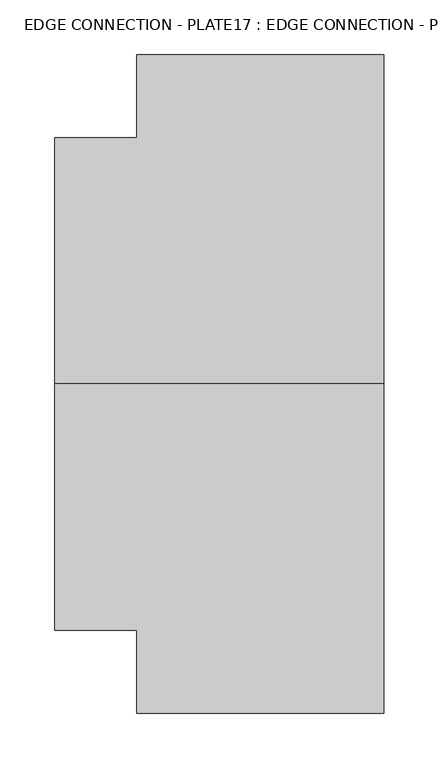
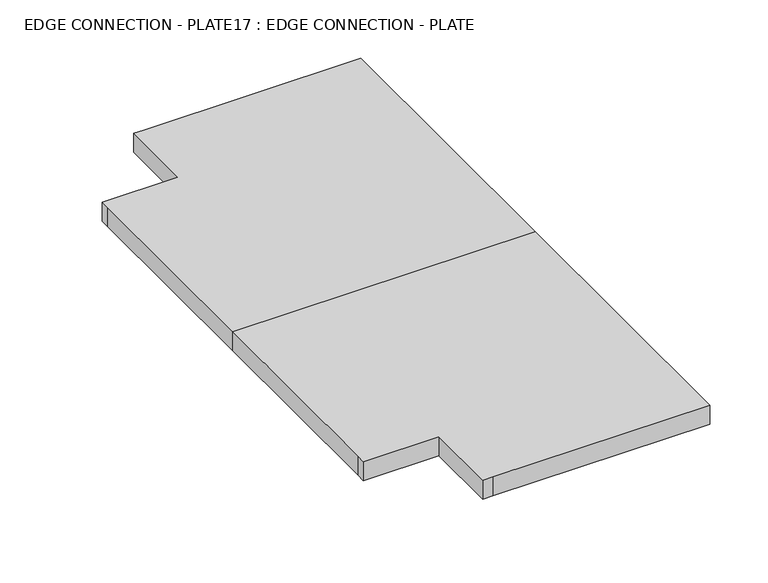
"""IFC4 building model written with IfcOpenShell, lengths in millimetres: fastener geometry, EDGE CONNECTION - PLATE17 : EDGE CONNECTION - PLATE."""

from ifc_helpers import new_model, si_unit, frame, origin, place, context, project, spatial, polyline, outline, extrude, source, transform, mapped, element, save


def edge_connection_plate17_edge_connection_plate_12cd6564(model_context):
    return source(origin(), model_context, "Body", "SweptSolid", [
        extrude(outline(polyline([(5700.0, 22499.5208589), (6000.0, 22499.5208589), (6000.0, 22199.5208589), (5784.862, 22199.5208589), (5774.862, 22199.5208589), (5774.862, 22275.0508589), (5700.0, 22275.0508589), (5700.0, 22285.0508589), (5700.0, 22499.5208589)])), frame((0.0, 0.0, 200.0), z_axis=(0.0, 0.0, 1.0), x_axis=(1.0, 0.0, 0.0)), (0.0, 0.0, 1.0), 20.0),
        extrude(outline(polyline([(5700.0, 22499.5208589), (5700.0, 22713.9908589), (5700.0, 22723.9908589), (5774.862, 22723.9908589), (5774.862, 22799.5208589), (5784.862, 22799.5208589), (6000.0, 22799.5208589), (6000.0, 22499.5208589), (5700.0, 22499.5208589)])), frame((0.0, 0.0, 200.0), z_axis=(0.0, 0.0, 1.0), x_axis=(1.0, 0.0, 0.0)), (0.0, 0.0, 1.0), 20.0),
    ])


if __name__ == "__main__":
    model = new_model("IFC4")
    model_context = context("Model", 3, world=origin())
    ifc_project = project(units=[si_unit("LENGTHUNIT", "METRE", prefix="MILLI")], contexts=[model_context])
    site = spatial("IfcSite", under=ifc_project)
    building = spatial("IfcBuilding", under=site)
    placement = place(None, origin())
    edge_connection_plate17_edge_connection_plate_shape = edge_connection_plate17_edge_connection_plate_12cd6564(model_context)
    element("IfcFastener", 1, ObjectType="EDGE CONNECTION - PLATE17 : EDGE CONNECTION - PLATE", at=placement, inside=building, context=model_context, shape_type="MappedRepresentation", body=[
        mapped(edge_connection_plate17_edge_connection_plate_shape, transform((0.0, 0.0, 0.0), x_axis=(1.0, 0.0, 0.0), y_axis=(0.0, 1.0, 0.0), z_axis=(0.0, 0.0, 1.0))),
    ])
    save(model, "model.ifc")
